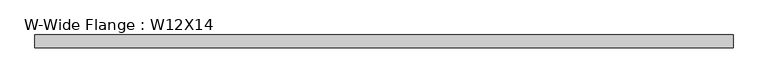
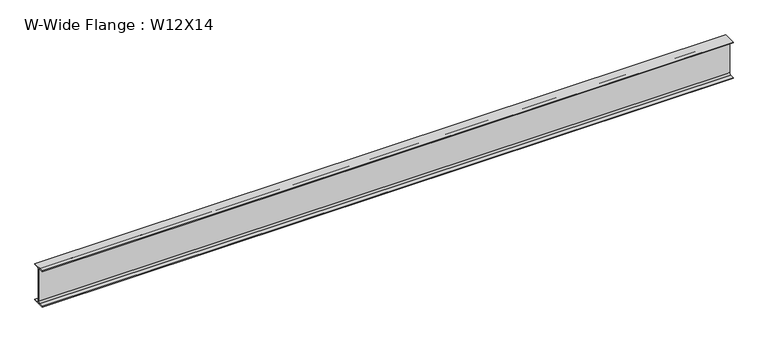
"""IFC4 building model written with IfcOpenShell, lengths in millimetres: beam geometry, W-Wide Flange : W12X14."""

from ifc_helpers import new_model, si_unit, point, frame, frame_2d, origin, place, context, project, spatial, polyline, circle_curve, trimmed, segment, composite_curve, outline, extrude, source, transform, mapped, element, save


def w_wide_flange_w12x14_7cca6224(model_context):
    return source(origin(), model_context, "Body", "SweptSolid", [
        extrude(outline(composite_curve([segment(polyline([(-50.419, -145.415), (-15.875, -145.415)]), True, "CONTINUOUS"), segment(trimmed(circle_curve(frame_2d((-15.875, -132.08)), 13.335), [point((-15.875, -145.415))], [point((-2.54, -132.08))], True, "CARTESIAN"), True, "CONTINUOUS"), segment(polyline([(-2.54, -132.08), (-2.54, 132.08)]), True, "CONTINUOUS"), segment(trimmed(circle_curve(frame_2d((-15.875, 132.08)), 13.335), [point((-2.54, 132.08))], [point((-15.875, 145.415))], True, "CARTESIAN"), True, "CONTINUOUS"), segment(polyline([(-15.875, 145.415), (-50.419, 145.415), (-50.419, 151.13), (50.419, 151.13), (50.419, 145.415), (15.875, 145.415)]), True, "CONTINUOUS"), segment(trimmed(circle_curve(frame_2d((15.875, 132.08)), 13.335), [point((15.875, 145.415))], [point((2.54, 132.08))], True, "CARTESIAN"), True, "CONTINUOUS"), segment(polyline([(2.54, 132.08), (2.54, -132.08)]), True, "CONTINUOUS"), segment(trimmed(circle_curve(frame_2d((15.875, -132.08)), 13.335), [point((2.54, -132.08))], [point((15.875, -145.415))], True, "CARTESIAN"), True, "CONTINUOUS"), segment(polyline([(15.875, -145.415), (50.419, -145.415), (50.419, -151.13), (-50.419, -151.13), (-50.419, -145.415)]), True, "CONTINUOUS")], self_intersect=False)), frame((-2731.008, 0.0, 0.0), z_axis=(1.0, 0.0, 0.0), x_axis=(0.0, 1.0, 0.0)), (0.0, 0.0, 1.0), 5474.081),
    ])


if __name__ == "__main__":
    model = new_model("IFC4")
    model_context = context("Model", 3, world=origin())
    ifc_project = project(units=[si_unit("LENGTHUNIT", "METRE", prefix="MILLI")], contexts=[model_context])
    site = spatial("IfcSite", under=ifc_project)
    building = spatial("IfcBuilding", under=site)
    placement = place(None, origin())
    w_wide_flange_w12x14_shape = w_wide_flange_w12x14_7cca6224(model_context)
    element("IfcBeam", 1, ObjectType="W-Wide Flange : W12X14", at=placement, inside=building, context=model_context, shape_type="MappedRepresentation", body=[
        mapped(w_wide_flange_w12x14_shape, transform((0.0, 0.0, 0.0), x_axis=(1.0, 0.0, 0.0), y_axis=(0.0, 1.0, 0.0), z_axis=(0.0, 0.0, 1.0))),
    ])
    save(model, "model.ifc")

# Revit data of these elements
# Type "W-Wide Flange : W12X14"
#   Assembly Code = "B10"
#   W = 14
#   Length [instance default] = 5' - 0"
#   bf = 0' - 3.97"
#   d = 0' - 11.9"
#   k = 0' - 0 3/4"
#   k2 = 0' - 0.525"
#   tf = 0' - 0.225"
#   tw = 0' - 0.2"
#   A = 0.0288889 SF
#   Structural Material [instance default] = Steel ASTM A992
# Element 1 (IfcBeam, "W-Wide Flange : W12X14")
#   Materials on its faces: "Steel ASTM A992"
# Materials
#   "Steel ASTM A992": class "Metal", colour RGB 199 199 199, transparency 0, Description = "Structural steel 50ksi", Cost = 0
